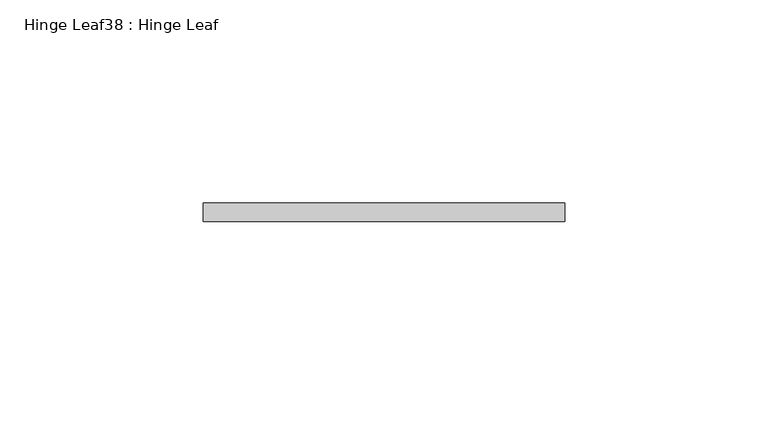
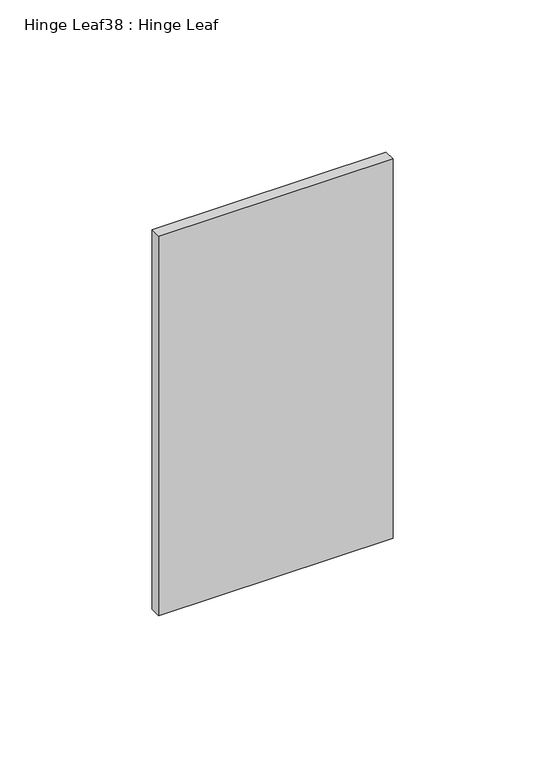
"""IFC4 building model written with IfcOpenShell, lengths in millimetres: proxy geometry, Hinge Leaf38 : Hinge Leaf."""

from ifc_helpers import new_model, si_unit, frame, origin, place, context, project, spatial, polyline, outline, extrude, source, transform, mapped, element, save


def hinge_leaf38_hinge_leaf_d7f0489c(model_context):
    return source(origin(), model_context, "Body", "SweptSolid", [
        extrude(outline(polyline([(587327.7934739, -534104.7943841), (587416.6934739, -534104.7943841), (587416.6934739, -534109.3663841), (587327.7934739, -534109.3663841), (587327.7934739, -534104.7943841)])), frame((0.0, 0.0, 311.15), z_axis=(0.0, 0.0, 1.0), x_axis=(1.0, 0.0, 0.0)), (0.0, 0.0, 1.0), 152.4),
    ])


if __name__ == "__main__":
    model = new_model("IFC4")
    model_context = context("Model", 3, world=origin())
    ifc_project = project(units=[si_unit("LENGTHUNIT", "METRE", prefix="MILLI")], contexts=[model_context])
    site = spatial("IfcSite", under=ifc_project)
    building = spatial("IfcBuilding", under=site)
    placement = place(None, origin())
    hinge_leaf38_hinge_leaf_shape = hinge_leaf38_hinge_leaf_d7f0489c(model_context)
    element("IfcBuildingElementProxy", 1, Name="Hinge Leaf38 : Hinge Leaf", ObjectType="Hinge Leaf38 : Hinge Leaf", at=placement, inside=building, context=model_context, shape_type="MappedRepresentation", body=[
        mapped(hinge_leaf38_hinge_leaf_shape, transform((0.0, 0.0, 0.0), x_axis=(1.0, 0.0, 0.0), y_axis=(0.0, 1.0, 0.0), z_axis=(0.0, 0.0, 1.0))),
    ])
    save(model, "model.ifc")

# Revit data of these elements
# Element 1 (IfcBuildingElementProxy, "Hinge Leaf38 : Hinge Leaf")
#   Materials on its faces: "6\"X6\" WELD-ON STL BUTT HINGE"
# Materials
#   "6\"X6\" WELD-ON STL BUTT HINGE": class "Metal", colour RGB 189 187 185, transparency 0, Description = "Carbon steel", Cost = 0
